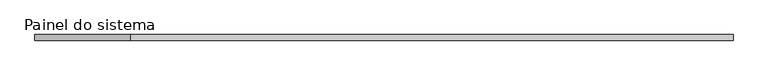
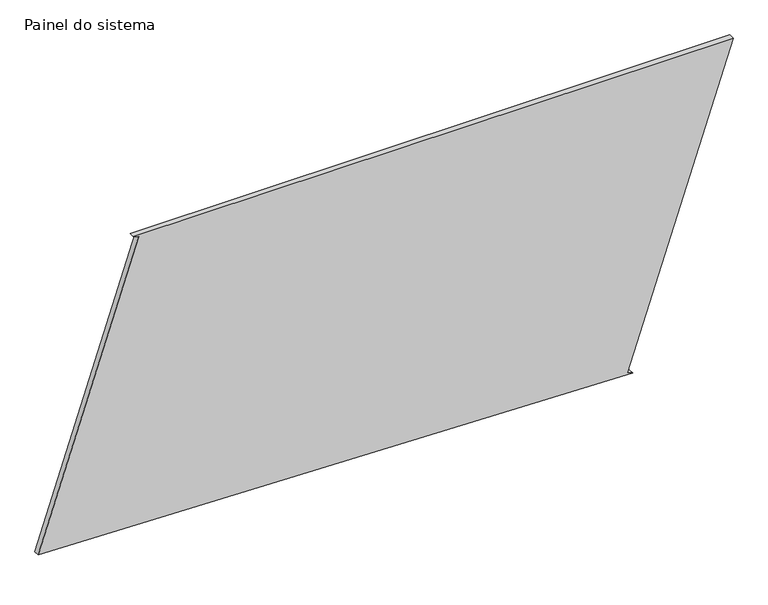
"""IFC4 building model written with IfcOpenShell, lengths in millimetres: plate geometry, Painel do sistema : Envidraçado."""

from ifc_helpers import new_model, si_unit, frame, origin, place, context, project, spatial, polyline, outline, extrude, source, transform, mapped, element, save


def painel_do_sistema_535277ac(model_context):
    return source(origin(), model_context, "Body", "SweptSolid", [
        extrude(outline(polyline([(0.0, 1106.2089665), (7.8961296, 1082.488698), (1429.1896696, 1555.6164812), (1429.1896696, -1129.4595122), (1421.2935399, -1105.7392437), (69.8455081, -1555.6164812), (0.0, 1106.2089665)])), frame((0.0, 24.5, 0.0), z_axis=(0.0, 1.0, 0.0), x_axis=(0.0, 0.0, 1.0)), (0.0, 0.0, 1.0), 25.0),
    ])


if __name__ == "__main__":
    model = new_model("IFC4")
    model_context = context("Model", 3, world=origin())
    ifc_project = project(units=[si_unit("LENGTHUNIT", "METRE", prefix="MILLI")], contexts=[model_context])
    site = spatial("IfcSite", under=ifc_project)
    building = spatial("IfcBuilding", under=site)
    placement = place(None, origin())
    painel_do_sistema_shape = painel_do_sistema_535277ac(model_context)
    element("IfcPlate", 1, ObjectType="Painel do sistema : Envidraçado", at=placement, inside=building, context=model_context, shape_type="MappedRepresentation", body=[
        mapped(painel_do_sistema_shape, transform((0.0, 0.0, 0.0), x_axis=(1.0, 0.0, 0.0), y_axis=(0.0, 1.0, 0.0), z_axis=(0.0, 0.0, 1.0))),
    ])
    save(model, "model.ifc")

# Revit data of these elements
# Type "Painel do sistema : Envidraçado"
#   Construction Type Id = "GSP4R"
#   Analytic Construction = "Vidraça única Pilkington 1/8 pol"
#   Visual Light Transmittance = 0.9
#   Solar Heat Gain Coefficient = 0.86
#   Heat Transfer Coefficient (U) = 6.7069 W/(m²·K)
# Element 1 (IfcPlate, "Painel do sistema : Envidraçado")
#   Materials on its faces: "Vidro"
# Materials
#   "Vidro": class "Vidro", colour RGB 0 128 192, transparency 0.9, Description = "Vidro de sílica", Cost = 0
